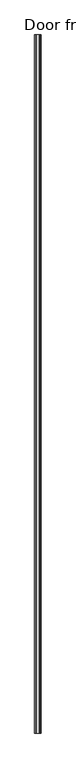
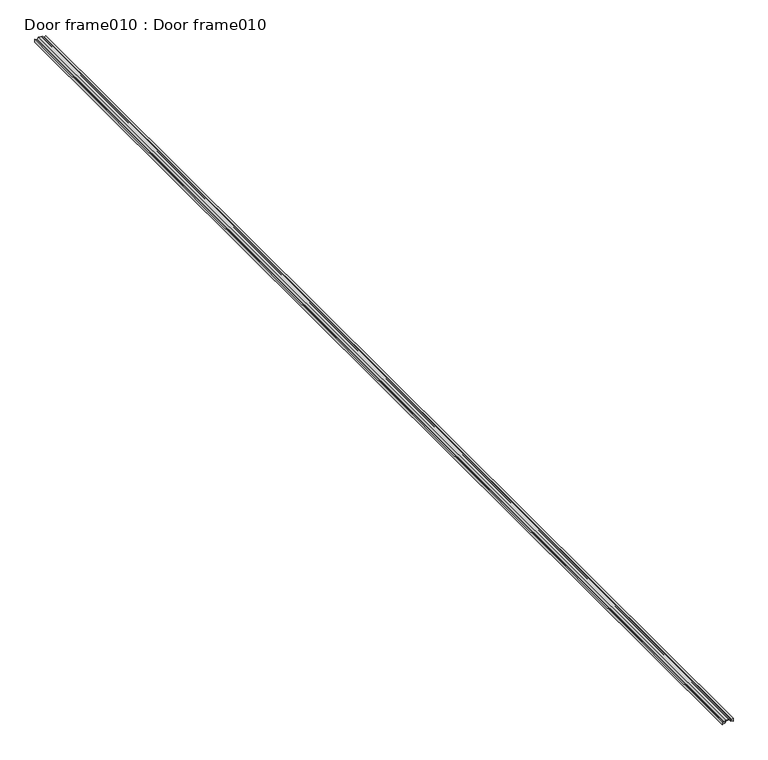
"""IFC4 building model written with IfcOpenShell, lengths in millimetres: proxy geometry, Door frame010 : Door frame010."""

import ifcopenshell
import ifcopenshell.guid

model = None  # the IFC model being written
_history = None  # IfcOwnerHistory: only IFC2X3 demands one
_inside = {}  # id of a spatial element -> (the spatial element, [elements in it])
_under = {}  # id of a project, library or spatial element -> (it, [spatial elements below it])
_declared = {}  # id of a project -> (the project, [libraries it declares])
_typed = {}  # id of a type object -> (the type object, [elements of that type])
_made_of = {}  # id of a material, layer set ... -> (it, [elements and type objects made of it])


def new_model(schema):
    """Start an empty IFC model of exactly this schema.

    Asked for "IFC4X3", IfcOpenShell would pick the latest addendum, in which some entities
    have other attributes; the version numbers below select the first issue.
    IFC2X3 requires an IfcOwnerHistory on every rooted entity: one is made here for all.
    """
    global model, _history
    if schema == "IFC4X3":
        model = ifcopenshell.file(schema_version=(4, 3, 0, 0))
    else:
        model = ifcopenshell.file(schema=schema)
    _inside.clear()
    _under.clear()
    _declared.clear()
    _typed.clear()
    _made_of.clear()
    _history = None
    if model.schema == "IFC2X3":
        org = make("IfcOrganization", Name="unknown")
        user = make(
            "IfcPersonAndOrganization",
            ThePerson=make("IfcPerson", FamilyName="unknown"),
            TheOrganization=org,
        )
        app = make(
            "IfcApplication",
            ApplicationDeveloper=org,
            Version="unknown",
            ApplicationFullName="unknown",
            ApplicationIdentifier="unknown",
        )
        _history = make(
            "IfcOwnerHistory",
            OwningUser=user,
            OwningApplication=app,
            ChangeAction="ADDED",
            CreationDate=0,
        )
    return model


def make(cls, **values):
    """One entity of the class cls with the attributes given. An attribute that is None is left unset."""
    return model.create_entity(
        cls, **{name: value for name, value in values.items() if value is not None}
    )


def rooted(cls, **values):
    """An entity with a GlobalId (a new one), such as an element, a storey or a relation."""
    return make(cls, GlobalId=ifcopenshell.guid.new(), OwnerHistory=_history, **values)


def si_unit(unit_type, name, prefix=None):
    """IfcSIUnit, for example si_unit("LENGTHUNIT", "METRE", prefix="MILLI")."""
    return make("IfcSIUnit", UnitType=unit_type, Prefix=prefix, Name=name)


def assignment(units):
    """IfcUnitAssignment: the units of a project."""
    return None if units is None else make("IfcUnitAssignment", Units=units)


def point(xyz):
    """IfcCartesianPoint."""
    return None if xyz is None else make("IfcCartesianPoint", Coordinates=xyz)


def direction(xyz):
    """IfcDirection."""
    return None if xyz is None else make("IfcDirection", DirectionRatios=xyz)


def frame(location, z_axis=None, x_axis=None):
    """IfcAxis2Placement3D, a coordinate frame: its origin and axes. An axis left out is left unset."""
    return make(
        "IfcAxis2Placement3D",
        Location=point(location),
        Axis=direction(z_axis),
        RefDirection=direction(x_axis),
    )


def origin():
    """The frame at (0, 0, 0) with its axes left unset."""
    return frame((0.0, 0.0, 0.0))


def place(relative_to, where):
    """IfcLocalPlacement: puts the frame where relative to a parent placement (None: the world)."""
    return make(
        "IfcLocalPlacement", PlacementRelTo=relative_to, RelativePlacement=where
    )


def context(
    kind, dimensions, precision=None, world=None, true_north=None, identifier=None
):
    """IfcGeometricRepresentationContext, for example the 3D "Model" context."""
    return make(
        "IfcGeometricRepresentationContext",
        ContextIdentifier=identifier,
        ContextType=kind,
        CoordinateSpaceDimension=dimensions,
        Precision=precision,
        WorldCoordinateSystem=world,
        TrueNorth=true_north,
    )


def project(units=None, contexts=None):
    """IfcProject with its units and contexts."""
    return rooted(
        "IfcProject",
        Name="project",
        RepresentationContexts=contexts,
        UnitsInContext=assignment(units),
    )


def spatial(cls, under=None, at=None, **own):
    """A site, building, storey or space (cls), placed at a placement, below another one or the project."""
    s = rooted(cls, ObjectPlacement=at, **own)
    if under is not None:
        _under.setdefault(under.id(), (under, []))[1].append(s)
    return s


def polyline(points):
    """IfcPolyline through the points."""
    return make("IfcPolyline", Points=[point(p) for p in points])


def outline(outer, holes=None, kind="AREA"):
    """IfcArbitraryClosedProfileDef: a profile drawn as a closed curve; with holes, ...WithVoids."""
    if holes is None:
        return make("IfcArbitraryClosedProfileDef", ProfileType=kind, OuterCurve=outer)
    return make(
        "IfcArbitraryProfileDefWithVoids",
        ProfileType=kind,
        OuterCurve=outer,
        InnerCurves=holes,
    )


def extrude(swept, where, along, depth):
    """IfcExtrudedAreaSolid: the profile swept, set in the frame where, extruded along a direction by depth."""
    return make(
        "IfcExtrudedAreaSolid",
        SweptArea=swept,
        Position=where,
        ExtrudedDirection=direction(along),
        Depth=depth,
    )


def shape(context_of_items, identifier, shape_type, items):
    """IfcShapeRepresentation: the items that make up one representation, for example the "Body"."""
    return make(
        "IfcShapeRepresentation",
        ContextOfItems=context_of_items,
        RepresentationIdentifier=identifier,
        RepresentationType=shape_type,
        Items=items,
    )


def source(mapping_origin, context_of_items, identifier, shape_type, items):
    """IfcRepresentationMap: a shape defined once, which mapped items show again and again."""
    return make(
        "IfcRepresentationMap",
        MappingOrigin=mapping_origin,
        MappedRepresentation=shape(context_of_items, identifier, shape_type, items),
    )


def transform(
    local_origin,
    x_axis=None,
    y_axis=None,
    z_axis=None,
    scale=None,
    scale2=None,
    scale3=None,
    uniform=True,
):
    """IfcCartesianTransformationOperator3D, or its non-uniform kind. x_axis, y_axis, z_axis: its Axis1, 2, 3."""
    if uniform:
        return make(
            "IfcCartesianTransformationOperator3D",
            Axis1=direction(x_axis),
            Axis2=direction(y_axis),
            LocalOrigin=point(local_origin),
            Scale=scale,
            Axis3=direction(z_axis),
        )
    return make(
        "IfcCartesianTransformationOperator3DnonUniform",
        Axis1=direction(x_axis),
        Axis2=direction(y_axis),
        LocalOrigin=point(local_origin),
        Scale=scale,
        Axis3=direction(z_axis),
        Scale2=scale2,
        Scale3=scale3,
    )


def mapped(mapping_source, mapping_target):
    """IfcMappedItem: shows the shape of a source again, moved by a transform."""
    return make(
        "IfcMappedItem", MappingSource=mapping_source, MappingTarget=mapping_target
    )


def made_of(thing, what):
    """Note that an element or type object is made of a material, layer set ...; save() writes the relation."""
    if what is not None:
        _made_of.setdefault(what.id(), (what, []))[1].append(thing)
    return thing


def element(
    cls,
    number,
    at=None,
    inside=None,
    cuts=None,
    type_object=None,
    material=None,
    context=None,
    identifier="Body",
    shape_type=None,
    held_by="IfcProductDefinitionShape",
    body=None,
    shapes=None,
    **own,
):
    """One element of the class cls, such as IfcWall. Its Tag is "e" and its number.

    at: its placement. inside: the storey or other place that contains it. cuts: it is an
    opening in that element (IfcRelVoidsElement). A single representation is given by context,
    identifier, shape_type and body (its items); several are given by shapes. held_by: the class
    of the entity that holds the representations. save() writes the other relations.
    """
    e = rooted(cls, Tag="e%d" % number, ObjectPlacement=at, **own)
    if body is not None:
        shapes = [shape(context, identifier, shape_type, body)]
    if shapes is not None:
        e.Representation = make(held_by, Representations=shapes)
    if inside is not None:
        _inside.setdefault(inside.id(), (inside, []))[1].append(e)
    if cuts is not None:
        rooted(
            "IfcRelVoidsElement", RelatingBuildingElement=cuts, RelatedOpeningElement=e
        )
    if type_object is not None:
        _typed.setdefault(type_object.id(), (type_object, []))[1].append(e)
    return made_of(e, material)


def aggregate(whole, parts):
    """IfcRelAggregates: a whole, such as a stair, and the parts it consists of."""
    return rooted("IfcRelAggregates", RelatingObject=whole, RelatedObjects=parts)


def save(model, path):
    """Write the relations noted so far, then the file.

    IfcRelAggregates (storeys below a building ...), IfcRelContainedInSpatialStructure (elements
    in a storey), IfcRelDefinesByType, IfcRelAssociatesMaterial and IfcRelDeclares: one each for
    every whole, place, type object, material and project.
    """
    for whole, parts in _under.values():
        aggregate(whole, parts)
    for where, things in _inside.values():
        rooted(
            "IfcRelContainedInSpatialStructure",
            RelatedElements=things,
            RelatingStructure=where,
        )
    for kind, things in _typed.values():
        rooted("IfcRelDefinesByType", RelatedObjects=things, RelatingType=kind)
    for what, things in _made_of.values():
        rooted("IfcRelAssociatesMaterial", RelatedObjects=things, RelatingMaterial=what)
    for by, libraries in _declared.values():
        rooted("IfcRelDeclares", RelatingContext=by, RelatedDefinitions=libraries)
    model.write(path)


def door_frame010_door_frame010_dc68b2cc(model_context):
    return source(origin(), model_context, "Body", "SweptSolid", [
        extrude(outline(polyline([(36662.6580816, 15538.4954576), (36662.6580816, 15540.1419606), (36665.8580816, 15542.3826247), (36665.8580816, 15547.7313685), (36662.6580816, 15549.9720326), (36662.6580816, 15551.6185356), (36661.1287449, 15554.2674246), (36665.9874184, 15554.2674246), (36664.4580816, 15551.6185356), (36664.4580816, 15550.6648984), (36667.4580816, 15548.5642757), (36667.4580816, 15541.5497174), (36664.4580816, 15539.4490948), (36664.4580816, 15538.4954576), (36666.0170308, 15535.7952784), (36661.0991325, 15535.7952784), (36662.6580816, 15538.4954576)])), frame((0.0, -1052.8906567, 0.0), z_axis=(0.0, 1.0, 0.0), x_axis=(0.0, 0.0, 1.0)), (0.0, 0.0, 1.0), 1999.85),
    ])


if __name__ == "__main__":
    model = new_model("IFC4")
    model_context = context("Model", 3, world=origin())
    ifc_project = project(units=[si_unit("LENGTHUNIT", "METRE", prefix="MILLI")], contexts=[model_context])
    site = spatial("IfcSite", under=ifc_project)
    building = spatial("IfcBuilding", under=site)
    placement = place(None, origin())
    door_frame010_door_frame010_shape = door_frame010_door_frame010_dc68b2cc(model_context)
    element("IfcBuildingElementProxy", 1, Name="Door frame010 : Door frame010", ObjectType="Door frame010 : Door frame010", at=placement, inside=building, context=model_context, shape_type="MappedRepresentation", body=[
        mapped(door_frame010_door_frame010_shape, transform((0.0, 0.0, 0.0), x_axis=(1.0, 0.0, 0.0), y_axis=(0.0, 1.0, 0.0), z_axis=(0.0, 0.0, 1.0))),
    ])
    save(model, "model.ifc")

# Revit data of these elements
# Type "Door frame010 : Door frame010"
#   NameOverride = "Door frame010"
# Element 1 (IfcBuildingElementProxy, "Door frame010 : Door frame010")
#   Materials on its faces: "FLEETWOOD SERIES T-3200 SINGLE SWING DOOR FRAME"
# Materials
#   "FLEETWOOD SERIES T-3200 SINGLE SWING DOOR FRAME": class "Unassigned", colour RGB 128 128 128, transparency 0, Cost = 0
